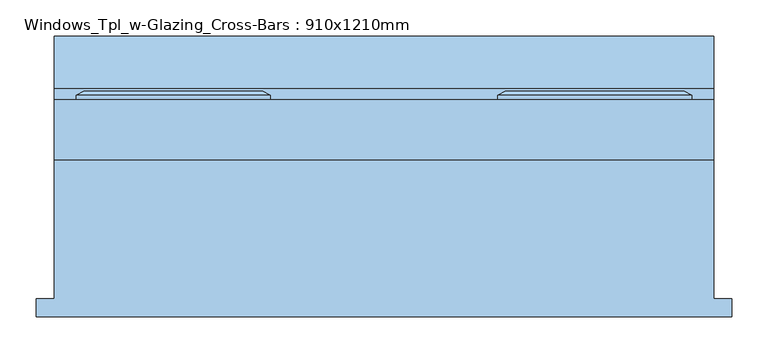
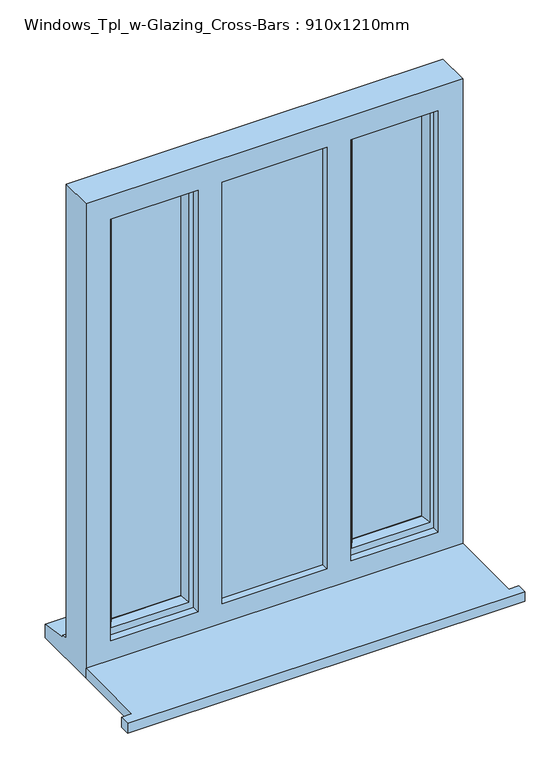
"""IFC4 building model written with IfcOpenShell, lengths in millimetres: window geometry, Windows_Tpl_w-Glazing_Cross-Bars : 910x1210mm."""

import ifcopenshell
import ifcopenshell.guid

model = None  # the IFC model being written
_history = None  # IfcOwnerHistory: only IFC2X3 demands one
_inside = {}  # id of a spatial element -> (the spatial element, [elements in it])
_under = {}  # id of a project, library or spatial element -> (it, [spatial elements below it])
_declared = {}  # id of a project -> (the project, [libraries it declares])
_typed = {}  # id of a type object -> (the type object, [elements of that type])
_made_of = {}  # id of a material, layer set ... -> (it, [elements and type objects made of it])


def new_model(schema):
    """Start an empty IFC model of exactly this schema.

    Asked for "IFC4X3", IfcOpenShell would pick the latest addendum, in which some entities
    have other attributes; the version numbers below select the first issue.
    IFC2X3 requires an IfcOwnerHistory on every rooted entity: one is made here for all.
    """
    global model, _history
    if schema == "IFC4X3":
        model = ifcopenshell.file(schema_version=(4, 3, 0, 0))
    else:
        model = ifcopenshell.file(schema=schema)
    _inside.clear()
    _under.clear()
    _declared.clear()
    _typed.clear()
    _made_of.clear()
    _history = None
    if model.schema == "IFC2X3":
        org = make("IfcOrganization", Name="unknown")
        user = make(
            "IfcPersonAndOrganization",
            ThePerson=make("IfcPerson", FamilyName="unknown"),
            TheOrganization=org,
        )
        app = make(
            "IfcApplication",
            ApplicationDeveloper=org,
            Version="unknown",
            ApplicationFullName="unknown",
            ApplicationIdentifier="unknown",
        )
        _history = make(
            "IfcOwnerHistory",
            OwningUser=user,
            OwningApplication=app,
            ChangeAction="ADDED",
            CreationDate=0,
        )
    return model


def make(cls, **values):
    """One entity of the class cls with the attributes given. An attribute that is None is left unset."""
    return model.create_entity(
        cls, **{name: value for name, value in values.items() if value is not None}
    )


def rooted(cls, **values):
    """An entity with a GlobalId (a new one), such as an element, a storey or a relation."""
    return make(cls, GlobalId=ifcopenshell.guid.new(), OwnerHistory=_history, **values)


def si_unit(unit_type, name, prefix=None):
    """IfcSIUnit, for example si_unit("LENGTHUNIT", "METRE", prefix="MILLI")."""
    return make("IfcSIUnit", UnitType=unit_type, Prefix=prefix, Name=name)


def assignment(units):
    """IfcUnitAssignment: the units of a project."""
    return None if units is None else make("IfcUnitAssignment", Units=units)


def point(xyz):
    """IfcCartesianPoint."""
    return None if xyz is None else make("IfcCartesianPoint", Coordinates=xyz)


def direction(xyz):
    """IfcDirection."""
    return None if xyz is None else make("IfcDirection", DirectionRatios=xyz)


def frame(location, z_axis=None, x_axis=None):
    """IfcAxis2Placement3D, a coordinate frame: its origin and axes. An axis left out is left unset."""
    return make(
        "IfcAxis2Placement3D",
        Location=point(location),
        Axis=direction(z_axis),
        RefDirection=direction(x_axis),
    )


def origin():
    """The frame at (0, 0, 0) with its axes left unset."""
    return frame((0.0, 0.0, 0.0))


def place(relative_to, where):
    """IfcLocalPlacement: puts the frame where relative to a parent placement (None: the world)."""
    return make(
        "IfcLocalPlacement", PlacementRelTo=relative_to, RelativePlacement=where
    )


def context(
    kind, dimensions, precision=None, world=None, true_north=None, identifier=None
):
    """IfcGeometricRepresentationContext, for example the 3D "Model" context."""
    return make(
        "IfcGeometricRepresentationContext",
        ContextIdentifier=identifier,
        ContextType=kind,
        CoordinateSpaceDimension=dimensions,
        Precision=precision,
        WorldCoordinateSystem=world,
        TrueNorth=true_north,
    )


def project(units=None, contexts=None):
    """IfcProject with its units and contexts."""
    return rooted(
        "IfcProject",
        Name="project",
        RepresentationContexts=contexts,
        UnitsInContext=assignment(units),
    )


def spatial(cls, under=None, at=None, **own):
    """A site, building, storey or space (cls), placed at a placement, below another one or the project."""
    s = rooted(cls, ObjectPlacement=at, **own)
    if under is not None:
        _under.setdefault(under.id(), (under, []))[1].append(s)
    return s


def polyline(points):
    """IfcPolyline through the points."""
    return make("IfcPolyline", Points=[point(p) for p in points])


def outline(outer, holes=None, kind="AREA"):
    """IfcArbitraryClosedProfileDef: a profile drawn as a closed curve; with holes, ...WithVoids."""
    if holes is None:
        return make("IfcArbitraryClosedProfileDef", ProfileType=kind, OuterCurve=outer)
    return make(
        "IfcArbitraryProfileDefWithVoids",
        ProfileType=kind,
        OuterCurve=outer,
        InnerCurves=holes,
    )


def extrude(swept, where, along, depth):
    """IfcExtrudedAreaSolid: the profile swept, set in the frame where, extruded along a direction by depth."""
    return make(
        "IfcExtrudedAreaSolid",
        SweptArea=swept,
        Position=where,
        ExtrudedDirection=direction(along),
        Depth=depth,
    )


def faces_of(points, faces, orient=None, outer=None):
    """IfcFace entities. A face is a list of loops; a loop is a list of indices into points, from 0.

    orient and outer hold one flag for each loop. By default every Orientation is true, the
    first loop of a face is its IfcFaceOuterBound and the others are IfcFaceBound.
    """
    made = []
    for i, loops in enumerate(faces):
        bounds = []
        for j, loop in enumerate(loops):
            is_outer = j == 0 if outer is None else outer[i][j]
            bounds.append(
                make(
                    "IfcFaceOuterBound" if is_outer else "IfcFaceBound",
                    Bound=make("IfcPolyLoop", Polygon=[points[k] for k in loop]),
                    Orientation=True if orient is None else orient[i][j],
                )
            )
        made.append(make("IfcFace", Bounds=bounds))
    return made


def faceted_brep(points, faces, orient=None, outer=None, voids=None):
    """IfcFacetedBrep: a solid bounded by flat faces; with voids (closed shells), ...WithVoids."""
    shared = [point(p) for p in points]
    hull = make("IfcClosedShell", CfsFaces=faces_of(shared, faces, orient, outer))
    if voids is None:
        return make("IfcFacetedBrep", Outer=hull)
    return make(
        "IfcFacetedBrepWithVoids",
        Outer=hull,
        Voids=[
            make(cls, CfsFaces=faces_of(shared, fs, o, b)) for cls, fs, o, b in voids
        ],
    )


def shape(context_of_items, identifier, shape_type, items):
    """IfcShapeRepresentation: the items that make up one representation, for example the "Body"."""
    return make(
        "IfcShapeRepresentation",
        ContextOfItems=context_of_items,
        RepresentationIdentifier=identifier,
        RepresentationType=shape_type,
        Items=items,
    )


def source(mapping_origin, context_of_items, identifier, shape_type, items):
    """IfcRepresentationMap: a shape defined once, which mapped items show again and again."""
    return make(
        "IfcRepresentationMap",
        MappingOrigin=mapping_origin,
        MappedRepresentation=shape(context_of_items, identifier, shape_type, items),
    )


def transform(
    local_origin,
    x_axis=None,
    y_axis=None,
    z_axis=None,
    scale=None,
    scale2=None,
    scale3=None,
    uniform=True,
):
    """IfcCartesianTransformationOperator3D, or its non-uniform kind. x_axis, y_axis, z_axis: its Axis1, 2, 3."""
    if uniform:
        return make(
            "IfcCartesianTransformationOperator3D",
            Axis1=direction(x_axis),
            Axis2=direction(y_axis),
            LocalOrigin=point(local_origin),
            Scale=scale,
            Axis3=direction(z_axis),
        )
    return make(
        "IfcCartesianTransformationOperator3DnonUniform",
        Axis1=direction(x_axis),
        Axis2=direction(y_axis),
        LocalOrigin=point(local_origin),
        Scale=scale,
        Axis3=direction(z_axis),
        Scale2=scale2,
        Scale3=scale3,
    )


def mapped(mapping_source, mapping_target):
    """IfcMappedItem: shows the shape of a source again, moved by a transform."""
    return make(
        "IfcMappedItem", MappingSource=mapping_source, MappingTarget=mapping_target
    )


def made_of(thing, what):
    """Note that an element or type object is made of a material, layer set ...; save() writes the relation."""
    if what is not None:
        _made_of.setdefault(what.id(), (what, []))[1].append(thing)
    return thing


def element(
    cls,
    number,
    at=None,
    inside=None,
    cuts=None,
    type_object=None,
    material=None,
    context=None,
    identifier="Body",
    shape_type=None,
    held_by="IfcProductDefinitionShape",
    body=None,
    shapes=None,
    **own,
):
    """One element of the class cls, such as IfcWall. Its Tag is "e" and its number.

    at: its placement. inside: the storey or other place that contains it. cuts: it is an
    opening in that element (IfcRelVoidsElement). A single representation is given by context,
    identifier, shape_type and body (its items); several are given by shapes. held_by: the class
    of the entity that holds the representations. save() writes the other relations.
    """
    e = rooted(cls, Tag="e%d" % number, ObjectPlacement=at, **own)
    if body is not None:
        shapes = [shape(context, identifier, shape_type, body)]
    if shapes is not None:
        e.Representation = make(held_by, Representations=shapes)
    if inside is not None:
        _inside.setdefault(inside.id(), (inside, []))[1].append(e)
    if cuts is not None:
        rooted(
            "IfcRelVoidsElement", RelatingBuildingElement=cuts, RelatedOpeningElement=e
        )
    if type_object is not None:
        _typed.setdefault(type_object.id(), (type_object, []))[1].append(e)
    return made_of(e, material)


def aggregate(whole, parts):
    """IfcRelAggregates: a whole, such as a stair, and the parts it consists of."""
    return rooted("IfcRelAggregates", RelatingObject=whole, RelatedObjects=parts)


def save(model, path):
    """Write the relations noted so far, then the file.

    IfcRelAggregates (storeys below a building ...), IfcRelContainedInSpatialStructure (elements
    in a storey), IfcRelDefinesByType, IfcRelAssociatesMaterial and IfcRelDeclares: one each for
    every whole, place, type object, material and project.
    """
    for whole, parts in _under.values():
        aggregate(whole, parts)
    for where, things in _inside.values():
        rooted(
            "IfcRelContainedInSpatialStructure",
            RelatedElements=things,
            RelatingStructure=where,
        )
    for kind, things in _typed.values():
        rooted("IfcRelDefinesByType", RelatedObjects=things, RelatingType=kind)
    for what, things in _made_of.values():
        rooted("IfcRelAssociatesMaterial", RelatedObjects=things, RelatingMaterial=what)
    for by, libraries in _declared.values():
        rooted("IfcRelDeclares", RelatingContext=by, RelatedDefinitions=libraries)
    model.write(path)


def windows_tpl_w_glazing_cross_bars_910x1210mm_b9cba8ba(model_context):
    return source(origin(), model_context, "Body", "SolidModel", [
        extrude(outline(polyline([(-906.6666667, -178.7934322), (-906.6666667, -153.7934322), (-881.6666667, -153.7934322), (-881.6666667, 37.7065678), (28.3333333, 37.7065678), (28.3333333, -153.7934322), (53.3333333, -153.7934322), (53.3333333, -178.7934322), (-906.6666667, -178.7934322)])), frame((0.0, 0.0, 900.0), z_axis=(0.0, 0.0, 1.0), x_axis=(1.0, 0.0, 0.0)), (0.0, 0.0, 1.0), 25.0),
        extrude(outline(polyline([(-623.3333333, 72.4565678), (-811.6666667, 72.4565678), (-811.6666667, 96.4565678), (-623.3333333, 96.4565678), (-623.3333333, 72.4565678)])), frame((0.0, 0.0, 993.0), z_axis=(0.0, 0.0, 1.0), x_axis=(1.0, 0.0, 0.0)), (0.0, 0.0, 1.0), 1047.0),
        extrude(outline(polyline([(-41.5186289, 72.4565678), (-230.1480377, 72.4565678), (-230.1480377, 96.4565678), (-41.5186289, 96.4565678), (-41.5186289, 72.4565678)])), frame((0.0, 0.0, 992.8519623), z_axis=(0.0, 0.0, 1.0), x_axis=(1.0, 0.0, 0.0)), (0.0, 0.0, 1.0), 1047.2960754),
        extrude(outline(polyline([(-563.3333333, 79.7065678), (-290.0, 79.7065678), (-290.0, 55.7065678), (-563.3333333, 55.7065678), (-563.3333333, 79.7065678)])), frame((0.0, 0.0, 963.0), z_axis=(0.0, 0.0, 1.0), x_axis=(1.0, 0.0, 0.0)), (0.0, 0.0, 1.0), 1107.0),
        faceted_brep([(28.3333333, 37.7065678, 2110.0), (-881.6666667, 37.7065678, 2110.0), (-881.6666667, 37.7065678, 900.0), (28.3333333, 37.7065678, 900.0), (-31.6666667, 37.7065678, 2050.0), (-31.6666667, 37.7065678, 975.0), (-242.0, 37.7065678, 975.0), (-242.0, 37.7065678, 2050.0), (-300.0, 37.7065678, 2050.0), (-300.0, 37.7065678, 975.0), (-553.3333333, 37.7065678, 975.0), (-553.3333333, 37.7065678, 2050.0), (-611.3333333, 37.7065678, 2050.0), (-611.3333333, 37.7065678, 975.0), (-821.6666667, 37.7065678, 975.0), (-821.6666667, 37.7065678, 2050.0), (-881.6666667, 120.7065678, 2110.0), (-881.6666667, 120.7065678, 951.0), (-881.6666667, 135.7065678, 949.68767), (-881.6666667, 135.7065678, 944.7449676), (-881.6666667, 208.2065678, 933.8088847), (-881.6666667, 208.2065678, 900.0), (28.3333333, 120.7065678, 2110.0), (28.3333333, 120.7065678, 951.0), (-841.6666667, 120.7065678, 2070.0), (-841.6666667, 120.7065678, 963.0), (-593.3333333, 120.7065678, 963.0), (-593.3333333, 120.7065678, 2070.0), (-553.3333333, 120.7065678, 2070.0), (-553.3333333, 120.7065678, 963.0), (-300.0, 120.7065678, 963.0), (-300.0, 120.7065678, 2070.0), (-260.0, 120.7065678, 2070.0), (-260.0, 120.7065678, 963.0), (-11.6666667, 120.7065678, 963.0), (-11.6666667, 120.7065678, 2070.0), (-841.6666667, 55.7065678, 2070.0), (-841.6666667, 55.7065678, 963.0), (-563.3333333, 55.7065678, 2070.0), (-290.0, 55.7065678, 2070.0), (-290.0, 55.7065678, 963.0), (-563.3333333, 55.7065678, 963.0), (-300.0, 55.7065678, 2050.0), (-553.3333333, 55.7065678, 2050.0), (-553.3333333, 55.7065678, 975.0), (-300.0, 55.7065678, 975.0), (-260.0, 55.7065678, 2070.0), (-11.6666667, 55.7065678, 2070.0), (-11.6666667, 55.7065678, 963.0), (-260.0, 55.7065678, 963.0), (-31.6666667, 55.7065678, 2050.0), (-242.0, 55.7065678, 2050.0), (-242.0, 55.7065678, 975.0), (-31.6666667, 55.7065678, 975.0), (-593.3333333, 55.7065678, 2070.0), (-593.3333333, 55.7065678, 963.0), (-611.3333333, 55.7065678, 2050.0), (-821.6666667, 55.7065678, 2050.0), (-821.6666667, 55.7065678, 975.0), (-611.3333333, 55.7065678, 975.0), (-553.3333333, 79.7065678, 2070.0), (-300.0, 79.7065678, 2070.0), (-290.0, 79.7065678, 2070.0), (-563.3333333, 79.7065678, 2070.0), (28.3333333, 208.2065678, 900.0), (28.3333333, 208.2065678, 933.8088847), (28.3333333, 135.7065678, 944.7449676), (28.3333333, 135.7065678, 949.68767), (-553.3333333, 79.7065678, 963.0), (-563.3333333, 79.7065678, 963.0), (-290.0, 79.7065678, 963.0), (-300.0, 79.7065678, 963.0)], [[[0, 1, 2, 3], [4, 5, 6, 7], [8, 9, 10, 11], [12, 13, 14, 15]], [[2, 1, 16, 17, 18, 19, 20, 21]], [[17, 16, 22, 23], [24, 25, 26, 27], [28, 29, 30, 31], [32, 33, 34, 35]], [[25, 24, 36, 37]], [[38, 39, 40, 41], [42, 43, 44, 45]], [[46, 47, 48, 49], [50, 51, 52, 53]], [[36, 54, 55, 37], [56, 57, 58, 59]], [[57, 15, 14, 58]], [[1, 0, 22, 16]], [[36, 24, 27, 54]], [[35, 47, 46, 32]], [[60, 28, 31, 61, 62, 39, 38, 63]], [[15, 57, 56, 12]], [[50, 4, 7, 51]], [[11, 43, 42, 8]], [[23, 22, 0, 3, 64, 65, 66, 67]], [[35, 34, 48, 47]], [[4, 50, 53, 5]], [[43, 11, 10, 44]], [[12, 56, 59, 13]], [[27, 26, 55, 54]], [[29, 28, 60, 68]], [[68, 60, 63, 69]], [[69, 63, 38, 41]], [[62, 70, 40, 39]], [[70, 62, 61, 71]], [[71, 61, 31, 30]], [[33, 32, 46, 49]], [[51, 7, 6, 52]], [[8, 42, 45, 9]], [[64, 3, 2, 21]], [[65, 64, 21, 20]], [[66, 65, 20, 19]], [[67, 66, 19, 18]], [[23, 67, 18, 17]], [[26, 25, 37, 55]], [[34, 33, 49, 48]], [[41, 40, 70, 71, 30, 29, 68, 69]], [[6, 5, 53, 52]], [[45, 44, 10, 9]], [[59, 58, 14, 13]]]),
        extrude(outline(polyline([(963.0, -436.6666667), (963.0, -416.6666667), (1506.5, -416.6666667), (1506.5, -290.0), (1526.5, -290.0), (1526.5, -416.6666667), (2070.0, -416.6666667), (2070.0, -436.6666667), (1526.5, -436.6666667), (1526.5, -563.3333333), (1506.5, -563.3333333), (1506.5, -436.6666667), (963.0, -436.6666667)])), frame((0.0, 63.7065678, 0.0), z_axis=(0.0, 1.0, 0.0), x_axis=(0.0, 0.0, 1.0)), (0.0, 0.0, 1.0), 8.0),
        extrude(outline(polyline([(993.0, -145.8333333), (993.0, -125.8333333), (1506.5, -125.8333333), (1506.5, -41.6666667), (1526.5, -41.6666667), (1526.5, -125.8333333), (2040.1480377, -125.8333333), (2040.1480377, -145.8333333), (1526.5, -145.8333333), (1526.5, -230.1480377), (1506.5, -230.1480377), (1506.5, -145.8333333), (993.0, -145.8333333)])), frame((0.0, 92.7065678, 0.0), z_axis=(0.0, 1.0, 0.0), x_axis=(0.0, 0.0, 1.0)), (0.0, 0.0, 1.0), 8.0),
        extrude(outline(polyline([(993.0, -727.5), (993.0, -707.5), (1506.5, -707.5), (1506.5, -623.3333333), (1526.5, -623.3333333), (1526.5, -707.5), (2040.1480377, -707.5), (2040.1480377, -727.5), (1526.5, -727.5), (1526.5, -811.6666667), (1506.5, -811.6666667), (1506.5, -727.5), (993.0, -727.5)])), frame((0.0, 92.7065678, 0.0), z_axis=(0.0, 1.0, 0.0), x_axis=(0.0, 0.0, 1.0)), (0.0, 0.0, 1.0), 8.0),
        faceted_brep([(-583.3333333, 120.7065678, 2080.0), (-583.3333333, 126.4800705, 2080.0), (-851.6666667, 126.4800705, 2080.0), (-851.6666667, 120.7065678, 2080.0), (-593.3333333, 55.7065678, 2070.0), (-593.3333333, 120.7065678, 2070.0), (-841.6666667, 120.7065678, 2070.0), (-841.6666667, 55.7065678, 2070.0), (-633.3333333, 70.1994677, 2030.0), (-623.1852956, 55.7065678, 2040.1480377), (-811.8147044, 55.7065678, 2040.1480377), (-801.6666667, 70.1994677, 2030.0), (-633.3333333, 84.7065678, 2030.0), (-801.6666667, 84.7065678, 2030.0), (-623.3333333, 108.7065678, 2040.0), (-623.3333333, 84.7065678, 2040.0), (-811.6666667, 84.7065678, 2040.0), (-811.6666667, 108.7065678, 2040.0), (-633.3333333, 126.4800705, 2030.0), (-633.3333333, 108.7065678, 2030.0), (-801.6666667, 108.7065678, 2030.0), (-801.6666667, 126.4800705, 2030.0), (-615.8875785, 132.2535732, 2047.4457548), (-819.1124215, 132.2535732, 2047.4457548), (-594.117943, 132.2535732, 2069.2153903), (-840.882057, 132.2535732, 2069.2153903), (-851.6666667, 126.4800705, 953.0), (-851.6666667, 120.7065678, 953.0), (-841.6666667, 120.7065678, 963.0), (-841.6666667, 55.7065678, 963.0), (-811.8147044, 55.7065678, 992.8519623), (-801.6666667, 70.1994677, 1003.0), (-801.6666667, 84.7065678, 1003.0), (-811.6666667, 84.7065678, 993.0), (-811.6666667, 108.7065678, 993.0), (-801.6666667, 108.7065678, 1003.0), (-801.6666667, 126.4800705, 1003.0), (-819.1124215, 132.2535732, 985.5542452), (-840.882057, 132.2535732, 963.7846097), (-583.3333333, 126.4800705, 953.0), (-583.3333333, 120.7065678, 953.0), (-593.3333333, 120.7065678, 963.0), (-593.3333333, 55.7065678, 963.0), (-623.1852956, 55.7065678, 992.8519623), (-633.3333333, 70.1994677, 1003.0), (-633.3333333, 84.7065678, 1003.0), (-623.3333333, 84.7065678, 993.0), (-623.3333333, 108.7065678, 993.0), (-633.3333333, 108.7065678, 1003.0), (-633.3333333, 126.4800705, 1003.0), (-615.8875785, 132.2535732, 985.5542452), (-594.117943, 132.2535732, 963.7846097)], [[[0, 1, 2, 3]], [[4, 5, 6, 7]], [[8, 9, 10, 11]], [[12, 8, 11, 13]], [[14, 15, 16, 17]], [[18, 19, 20, 21]], [[22, 18, 21, 23]], [[1, 24, 25, 2]], [[3, 2, 26, 27]], [[7, 6, 28, 29]], [[11, 10, 30, 31]], [[13, 11, 31, 32]], [[17, 16, 33, 34]], [[21, 20, 35, 36]], [[23, 21, 36, 37]], [[2, 25, 38, 26]], [[27, 26, 39, 40]], [[0, 3, 27, 40], [41, 28, 6, 5]], [[29, 28, 41, 42]], [[4, 7, 29, 42], [43, 30, 10, 9]], [[31, 30, 43, 44]], [[32, 31, 44, 45]], [[46, 33, 16, 15], [12, 13, 32, 45]], [[34, 33, 46, 47]], [[14, 17, 34, 47], [48, 35, 20, 19]], [[36, 35, 48, 49]], [[37, 36, 49, 50]], [[51, 38, 25, 24], [22, 23, 37, 50]], [[26, 38, 51, 39]], [[40, 39, 1, 0]], [[42, 41, 5, 4]], [[44, 43, 9, 8]], [[45, 44, 8, 12]], [[47, 46, 15, 14]], [[49, 48, 19, 18]], [[50, 49, 18, 22]], [[39, 51, 24, 1]]]),
        faceted_brep([(-270.0, 120.7065678, 2080.0), (-270.0, 126.4800705, 2080.0), (-270.0, 126.4800705, 953.0), (-270.0, 120.7065678, 953.0), (-260.0, 55.7065678, 2070.0), (-260.0, 120.7065678, 2070.0), (-260.0, 120.7065678, 963.0), (-260.0, 55.7065678, 963.0), (-220.0, 70.1994677, 2030.0), (-230.1480377, 55.7065678, 2040.1480377), (-230.1480377, 55.7065678, 992.8519623), (-220.0, 70.1994677, 1003.0), (-220.0, 84.7065678, 2030.0), (-220.0, 84.7065678, 1003.0), (-230.0, 108.7065678, 2040.0), (-230.0, 84.7065678, 2040.0), (-230.0, 84.7065678, 993.0), (-230.0, 108.7065678, 993.0), (-220.0, 126.4800705, 2030.0), (-220.0, 108.7065678, 2030.0), (-220.0, 108.7065678, 1003.0), (-220.0, 126.4800705, 1003.0), (-237.4457548, 132.2535732, 2047.4457548), (-237.4457548, 132.2535732, 985.5542452), (-259.2153903, 132.2535732, 2069.2153903), (-259.2153903, 132.2535732, 963.7846097), (-1.6666667, 126.4800705, 953.0), (-1.6666667, 120.7065678, 953.0), (-11.6666667, 120.7065678, 963.0), (-11.6666667, 55.7065678, 963.0), (-41.5186289, 55.7065678, 992.8519623), (-51.6666667, 70.1994677, 1003.0), (-51.6666667, 84.7065678, 1003.0), (-41.6666667, 84.7065678, 993.0), (-41.6666667, 108.7065678, 993.0), (-51.6666667, 108.7065678, 1003.0), (-51.6666667, 126.4800705, 1003.0), (-34.2209119, 132.2535732, 985.5542452), (-12.4512764, 132.2535732, 963.7846097), (-1.6666667, 126.4800705, 2080.0), (-1.6666667, 120.7065678, 2080.0), (-11.6666667, 120.7065678, 2070.0), (-11.6666667, 55.7065678, 2070.0), (-41.5186289, 55.7065678, 2040.1480377), (-51.6666667, 70.1994677, 2030.0), (-51.6666667, 84.7065678, 2030.0), (-41.6666667, 84.7065678, 2040.0), (-41.6666667, 108.7065678, 2040.0), (-51.6666667, 108.7065678, 2030.0), (-51.6666667, 126.4800705, 2030.0), (-34.2209119, 132.2535732, 2047.4457548), (-12.4512764, 132.2535732, 2069.2153903)], [[[0, 1, 2, 3]], [[4, 5, 6, 7]], [[8, 9, 10, 11]], [[12, 8, 11, 13]], [[14, 15, 16, 17]], [[18, 19, 20, 21]], [[22, 18, 21, 23]], [[1, 24, 25, 2]], [[3, 2, 26, 27]], [[7, 6, 28, 29]], [[11, 10, 30, 31]], [[13, 11, 31, 32]], [[17, 16, 33, 34]], [[21, 20, 35, 36]], [[23, 21, 36, 37]], [[2, 25, 38, 26]], [[27, 26, 39, 40]], [[29, 28, 41, 42]], [[31, 30, 43, 44]], [[32, 31, 44, 45]], [[34, 33, 46, 47]], [[36, 35, 48, 49]], [[37, 36, 49, 50]], [[26, 38, 51, 39]], [[40, 39, 1, 0]], [[3, 27, 40, 0], [5, 41, 28, 6]], [[42, 41, 5, 4]], [[7, 29, 42, 4], [9, 43, 30, 10]], [[44, 43, 9, 8]], [[45, 44, 8, 12]], [[15, 46, 33, 16], [13, 32, 45, 12]], [[47, 46, 15, 14]], [[17, 34, 47, 14], [19, 48, 35, 20]], [[49, 48, 19, 18]], [[50, 49, 18, 22]], [[24, 51, 38, 25], [23, 37, 50, 22]], [[39, 51, 24, 1]]]),
    ])


if __name__ == "__main__":
    model = new_model("IFC4")
    model_context = context("Model", 3, world=origin())
    ifc_project = project(units=[si_unit("LENGTHUNIT", "METRE", prefix="MILLI")], contexts=[model_context])
    site = spatial("IfcSite", under=ifc_project)
    building = spatial("IfcBuilding", under=site)
    placement = place(None, origin())
    windows_tpl_w_glazing_cross_bars_910x1210mm_shape = windows_tpl_w_glazing_cross_bars_910x1210mm_b9cba8ba(model_context)
    element("IfcWindow", 1, ObjectType="Windows_Tpl_w-Glazing_Cross-Bars : 910x1210mm", at=placement, inside=building, context=model_context, shape_type="MappedRepresentation", body=[
        mapped(windows_tpl_w_glazing_cross_bars_910x1210mm_shape, transform((0.0, 0.0, 0.0), x_axis=(1.0, 0.0, 0.0), y_axis=(0.0, 1.0, 0.0), z_axis=(0.0, 0.0, 1.0))),
    ])
    save(model, "model.ifc")

# Revit data of these elements
# Type "Windows_Tpl_w-Glazing_Cross-Bars : 910x1210mm"
#   Type Mark = "51"
#   Operation = "TriplePanelVertical"
#   Construction Type Id = "GSP4R"
#   Manufacturer = "Revit"
#   Keynote = "L10"
#   Analytic Construction = "1/8 in Pilkington single glazing"
#   Wrap Layers (Ext) from Ext = 102.5 mm
#   Wrap Layers (Int) from Ext = 177.5 mm
#   Window Board Projection = 25 mm
#   Window Board Extension = 25 mm
#   Visual Light Transmittance = 0.9
#   Solar Heat Gain Coefficient = 0.78
#   Rough Width = 910 mm
#   Rough Height = 1210 mm
#   Height = 1210 mm
#   Width = 910 mm
#   Heat Transfer Coefficient (U) = 3.6886 W/(m²·K)
#   Glazing Thickness = 24 mm
#   Glazing Bar Thickness = 20 mm
#   FrameOffset - External = 50 mm
#   Frame Depth = 65 mm
#   Default Head Height = 2110 mm
#   Cill Depth = 87.5 mm
#   Cavity Closer Width = 50 mm
#   Cavity Closer Offset from Ext = 102.5 mm
#   Cavity Closer Depth = 85 mm
#   Vis - Glazing Bars = yes
#   Vis - Cavity Closers = yes
#   Material Trim = Window Frame
#   Material Glazing Bars = Window Frame
#   Material Glass = Glass
#   Material Frame = Window Frame
#   Wall Closure = (empty or 0)
# Element 1 (IfcWindow, "Windows_Tpl_w-Glazing_Cross-Bars : 910x1210mm")
#   Materials on its faces: "Window Frame", "Glass"
# Materials
#   "Window Frame": class "Miscellaneous", colour RGB 249 249 249, transparency 0, Keynote = "L10"
#   "Glass": class "Glass", colour RGB 0 128 192, transparency 0.9, Description = "Soda Lime Glass", Cost = 0
